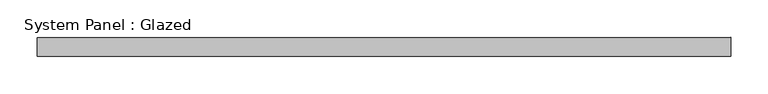
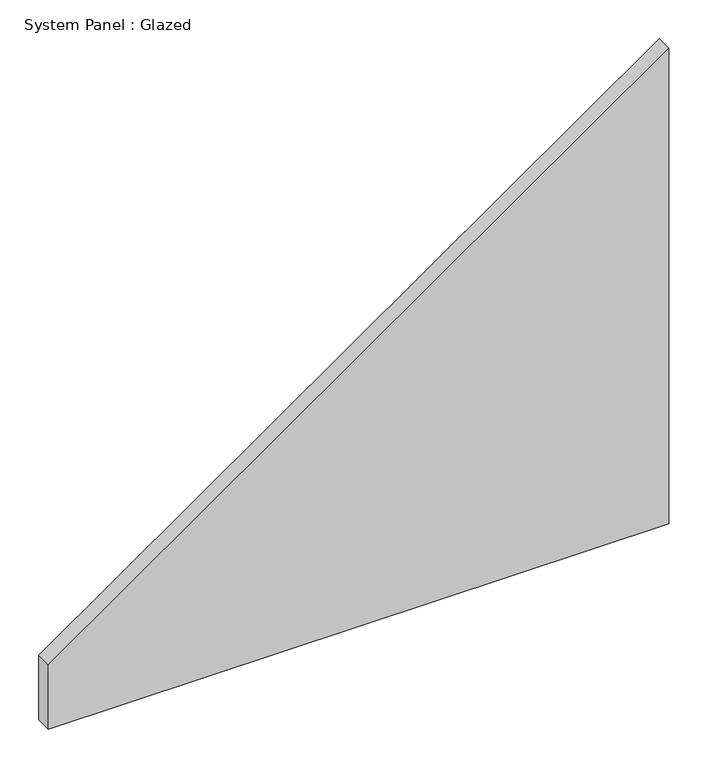
"""IFC4 building model written with IfcOpenShell, lengths in millimetres: plate geometry, System Panel : Glazed."""

from ifc_helpers import new_model, si_unit, frame, origin, place, context, project, spatial, polyline, outline, extrude, source, transform, mapped, element, save


def system_panel_glazed_fc82b317(model_context):
    return source(origin(), model_context, "Body", "SweptSolid", [
        extrude(outline(polyline([(0.0, -462.5), (0.0, 462.5), (749.3867239, 462.5), (101.694751, -462.5), (0.0, -462.5)])), frame((0.0, 24.5, 0.0), z_axis=(0.0, 1.0, 0.0), x_axis=(0.0, 0.0, 1.0)), (0.0, 0.0, 1.0), 25.0),
    ])


if __name__ == "__main__":
    model = new_model("IFC4")
    model_context = context("Model", 3, world=origin())
    ifc_project = project(units=[si_unit("LENGTHUNIT", "METRE", prefix="MILLI")], contexts=[model_context])
    site = spatial("IfcSite", under=ifc_project)
    building = spatial("IfcBuilding", under=site)
    placement = place(None, origin())
    system_panel_glazed_shape = system_panel_glazed_fc82b317(model_context)
    element("IfcPlate", 1, ObjectType="System Panel : Glazed", at=placement, inside=building, context=model_context, shape_type="MappedRepresentation", body=[
        mapped(system_panel_glazed_shape, transform((0.0, 0.0, 0.0), x_axis=(1.0, 0.0, 0.0), y_axis=(0.0, 1.0, 0.0), z_axis=(0.0, 0.0, 1.0))),
    ])
    save(model, "model.ifc")

# Revit data of these elements
# Type "System Panel : Glazed"
#   Construction Type Id = "GSP4R"
#   Analytic Construction = "1/8 in Pilkington single glazing"
#   Visual Light Transmittance = 0.9
#   Solar Heat Gain Coefficient = 0.86
#   Heat Transfer Coefficient (U) = 6.7069 W/(m²·K)
#   Define Thermal Properties by = 1
# Element 1 (IfcPlate, "System Panel : Glazed")
#   Materials on its faces: "Glass"
# Materials
#   "Glass": class "Glass", colour RGB 0 128 192, transparency 0.9, Description = "Soda Lime Glass", Cost = 0
